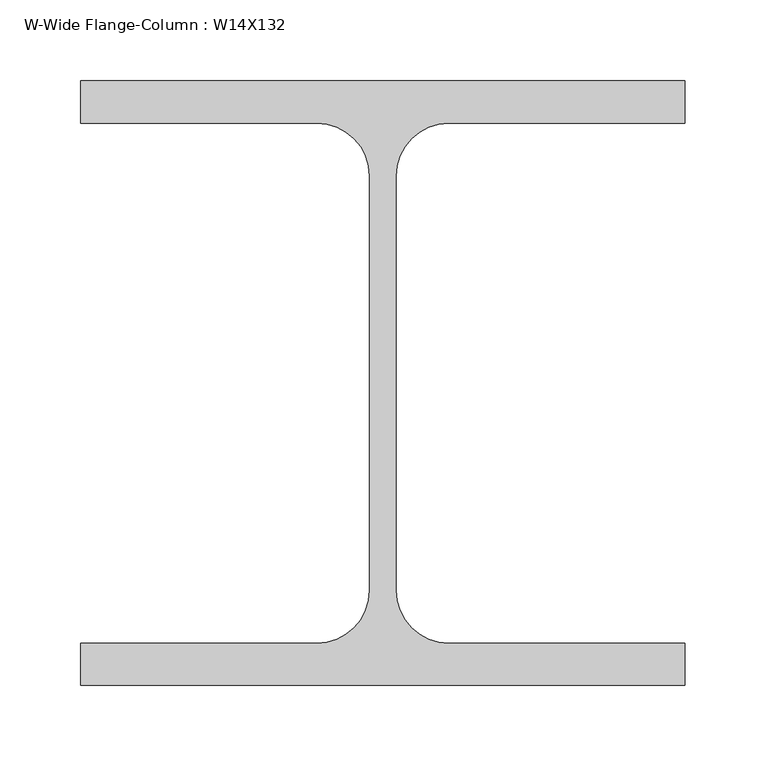
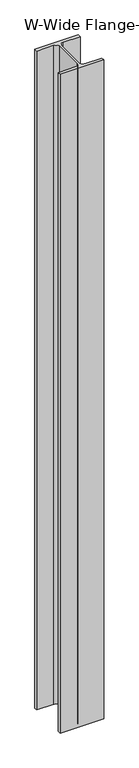
"""IFC4 building model written with IfcOpenShell, lengths in millimetres: column geometry, W-Wide Flange-Column : W14X132."""

from ifc_helpers import new_model, si_unit, point, frame_2d, origin, origin_with_axes, place, context, project, spatial, polyline, circle_curve, trimmed, segment, composite_curve, outline, extrude, source, transform, mapped, element, save


def w_wide_flange_column_w14x132_17457bbd(model_context):
    return source(origin(), model_context, "Body", "SweptSolid", [
        extrude(outline(composite_curve([segment(polyline([(186.69, 186.69), (186.69, 160.528), (40.767, 160.528)]), True, "CONTINUOUS"), segment(trimmed(circle_curve(frame_2d((40.767, 127.9525)), 32.5755), [point((40.767, 160.528))], [point((8.1915, 127.9525))], True, "CARTESIAN"), True, "CONTINUOUS"), segment(polyline([(8.1915, 127.9525), (8.1915, -127.9525)]), True, "CONTINUOUS"), segment(trimmed(circle_curve(frame_2d((40.767, -127.9525)), 32.5755), [point((8.1915, -127.9525))], [point((40.767, -160.528))], True, "CARTESIAN"), True, "CONTINUOUS"), segment(polyline([(40.767, -160.528), (186.69, -160.528), (186.69, -186.69), (-186.69, -186.69), (-186.69, -160.528), (-40.767, -160.528)]), True, "CONTINUOUS"), segment(trimmed(circle_curve(frame_2d((-40.767, -127.9525)), 32.5755), [point((-40.767, -160.528))], [point((-8.1915, -127.9525))], True, "CARTESIAN"), True, "CONTINUOUS"), segment(polyline([(-8.1915, -127.9525), (-8.1915, 127.9525)]), True, "CONTINUOUS"), segment(trimmed(circle_curve(frame_2d((-40.767, 127.9525)), 32.5755), [point((-8.1915, 127.9525))], [point((-40.767, 160.528))], True, "CARTESIAN"), True, "CONTINUOUS"), segment(polyline([(-40.767, 160.528), (-186.69, 160.528), (-186.69, 186.69), (186.69, 186.69)]), True, "CONTINUOUS")], self_intersect=False)), origin_with_axes(), (0.0, 0.0, 1.0), 5969.0),
    ])


if __name__ == "__main__":
    model = new_model("IFC4")
    model_context = context("Model", 3, world=origin())
    ifc_project = project(units=[si_unit("LENGTHUNIT", "METRE", prefix="MILLI")], contexts=[model_context])
    site = spatial("IfcSite", under=ifc_project)
    building = spatial("IfcBuilding", under=site)
    placement = place(None, origin())
    w_wide_flange_column_w14x132_shape = w_wide_flange_column_w14x132_17457bbd(model_context)
    element("IfcColumn", 1, ObjectType="W-Wide Flange-Column : W14X132", at=placement, inside=building, context=model_context, shape_type="MappedRepresentation", body=[
        mapped(w_wide_flange_column_w14x132_shape, transform((0.0, 0.0, 0.0), x_axis=(1.0, 0.0, 0.0), y_axis=(0.0, 1.0, 0.0), z_axis=(0.0, 0.0, 1.0))),
    ])
    save(model, "model.ifc")

# Revit data of these elements
# Type "W-Wide Flange-Column : W14X132"
#   Assembly Code = "B10"
#   W = 132
#   bf = 1' - 2.7"
#   d = 1' - 2.7"
#   k = 0' - 2 5/16"
#   kr = 0' - 1.2825"
#   tf = 0' - 1.03"
#   tw = 0' - 0.645"
#   A = 0.269444 SF
#   Column Material [instance default] = Metal - Steel - ASTM A992
# Element 1 (IfcColumn, "W-Wide Flange-Column : W14X132")
#   Materials on its faces: "Metal - Steel - ASTM A992"
# Materials
#   "Metal - Steel - ASTM A992": class "Metal", colour RGB 128 0 0, transparency 0
